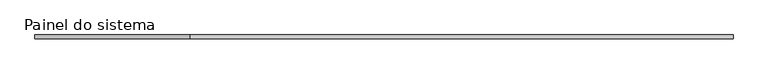
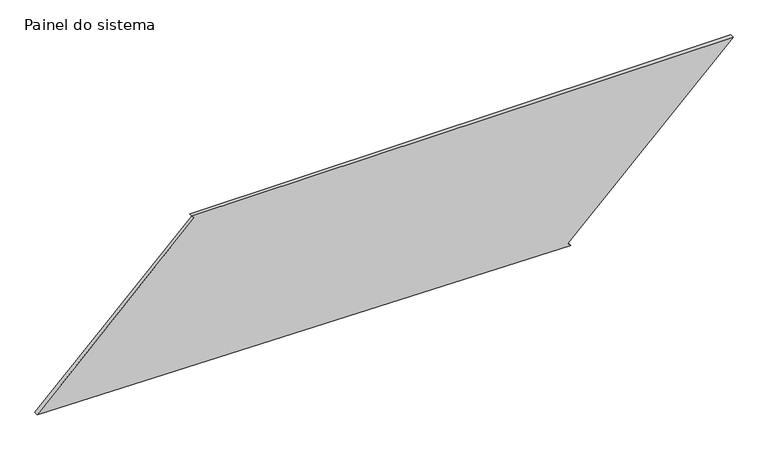
"""IFC4 building model written with IfcOpenShell, lengths in millimetres: plate geometry, Painel do sistema : Envidraçado."""

from ifc_helpers import new_model, si_unit, frame, origin, place, context, project, spatial, polyline, outline, extrude, source, transform, mapped, element, save


def painel_do_sistema_d099d1e2(model_context):
    return source(origin(), model_context, "Body", "SweptSolid", [
        extrude(outline(polyline([(0.0, 1250.8365048), (17.9061609, 1233.390319), (1103.0399544, 2347.1340632), (1103.0399544, -1303.5620846), (1085.1337934, -1286.1158987), (51.3711603, -2347.1340632), (0.0, 1250.8365048)])), frame((0.0, 24.5, 0.0), z_axis=(0.0, 1.0, 0.0), x_axis=(0.0, 0.0, 1.0)), (0.0, 0.0, 1.0), 25.0),
    ])


if __name__ == "__main__":
    model = new_model("IFC4")
    model_context = context("Model", 3, world=origin())
    ifc_project = project(units=[si_unit("LENGTHUNIT", "METRE", prefix="MILLI")], contexts=[model_context])
    site = spatial("IfcSite", under=ifc_project)
    building = spatial("IfcBuilding", under=site)
    placement = place(None, origin())
    painel_do_sistema_shape = painel_do_sistema_d099d1e2(model_context)
    element("IfcPlate", 1, ObjectType="Painel do sistema : Envidraçado", at=placement, inside=building, context=model_context, shape_type="MappedRepresentation", body=[
        mapped(painel_do_sistema_shape, transform((0.0, 0.0, 0.0), x_axis=(1.0, 0.0, 0.0), y_axis=(0.0, 1.0, 0.0), z_axis=(0.0, 0.0, 1.0))),
    ])
    save(model, "model.ifc")

# Revit data of these elements
# Type "Painel do sistema : Envidraçado"
#   Construction Type Id = "GSP4R"
#   Analytic Construction = "Vidraça única Pilkington 1/8 pol"
#   Visual Light Transmittance = 0.9
#   Solar Heat Gain Coefficient = 0.86
#   Heat Transfer Coefficient (U) = 6.7069 W/(m²·K)
# Element 1 (IfcPlate, "Painel do sistema : Envidraçado")
#   Materials on its faces: "Vidro"
# Materials
#   "Vidro": class "Vidro", colour RGB 0 128 192, transparency 0.9, Description = "Vidro de sílica", Cost = 0
